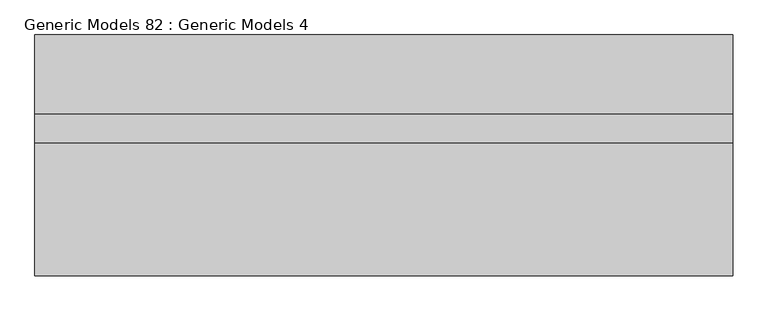
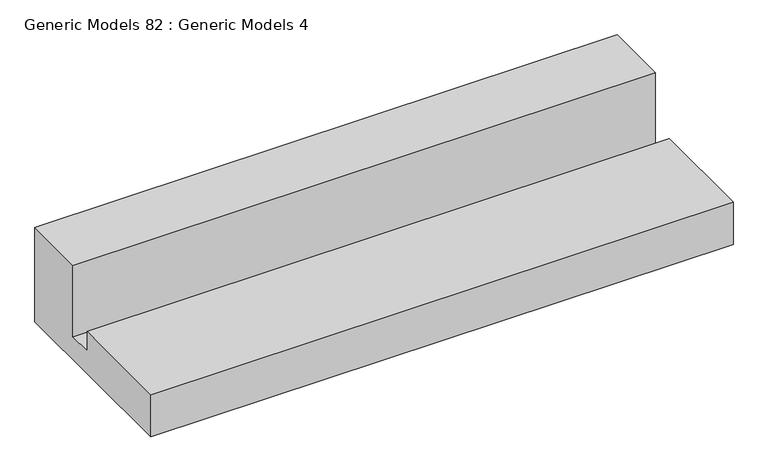
"""IFC4 building model written with IfcOpenShell, lengths in millimetres: proxy geometry, Generic Models 82 : Generic Models 4."""

import ifcopenshell
import ifcopenshell.guid

model = None  # the IFC model being written
_history = None  # IfcOwnerHistory: only IFC2X3 demands one
_inside = {}  # id of a spatial element -> (the spatial element, [elements in it])
_under = {}  # id of a project, library or spatial element -> (it, [spatial elements below it])
_declared = {}  # id of a project -> (the project, [libraries it declares])
_typed = {}  # id of a type object -> (the type object, [elements of that type])
_made_of = {}  # id of a material, layer set ... -> (it, [elements and type objects made of it])


def new_model(schema):
    """Start an empty IFC model of exactly this schema.

    Asked for "IFC4X3", IfcOpenShell would pick the latest addendum, in which some entities
    have other attributes; the version numbers below select the first issue.
    IFC2X3 requires an IfcOwnerHistory on every rooted entity: one is made here for all.
    """
    global model, _history
    if schema == "IFC4X3":
        model = ifcopenshell.file(schema_version=(4, 3, 0, 0))
    else:
        model = ifcopenshell.file(schema=schema)
    _inside.clear()
    _under.clear()
    _declared.clear()
    _typed.clear()
    _made_of.clear()
    _history = None
    if model.schema == "IFC2X3":
        org = make("IfcOrganization", Name="unknown")
        user = make(
            "IfcPersonAndOrganization",
            ThePerson=make("IfcPerson", FamilyName="unknown"),
            TheOrganization=org,
        )
        app = make(
            "IfcApplication",
            ApplicationDeveloper=org,
            Version="unknown",
            ApplicationFullName="unknown",
            ApplicationIdentifier="unknown",
        )
        _history = make(
            "IfcOwnerHistory",
            OwningUser=user,
            OwningApplication=app,
            ChangeAction="ADDED",
            CreationDate=0,
        )
    return model


def make(cls, **values):
    """One entity of the class cls with the attributes given. An attribute that is None is left unset."""
    return model.create_entity(
        cls, **{name: value for name, value in values.items() if value is not None}
    )


def rooted(cls, **values):
    """An entity with a GlobalId (a new one), such as an element, a storey or a relation."""
    return make(cls, GlobalId=ifcopenshell.guid.new(), OwnerHistory=_history, **values)


def si_unit(unit_type, name, prefix=None):
    """IfcSIUnit, for example si_unit("LENGTHUNIT", "METRE", prefix="MILLI")."""
    return make("IfcSIUnit", UnitType=unit_type, Prefix=prefix, Name=name)


def assignment(units):
    """IfcUnitAssignment: the units of a project."""
    return None if units is None else make("IfcUnitAssignment", Units=units)


def point(xyz):
    """IfcCartesianPoint."""
    return None if xyz is None else make("IfcCartesianPoint", Coordinates=xyz)


def direction(xyz):
    """IfcDirection."""
    return None if xyz is None else make("IfcDirection", DirectionRatios=xyz)


def frame(location, z_axis=None, x_axis=None):
    """IfcAxis2Placement3D, a coordinate frame: its origin and axes. An axis left out is left unset."""
    return make(
        "IfcAxis2Placement3D",
        Location=point(location),
        Axis=direction(z_axis),
        RefDirection=direction(x_axis),
    )


def origin():
    """The frame at (0, 0, 0) with its axes left unset."""
    return frame((0.0, 0.0, 0.0))


def place(relative_to, where):
    """IfcLocalPlacement: puts the frame where relative to a parent placement (None: the world)."""
    return make(
        "IfcLocalPlacement", PlacementRelTo=relative_to, RelativePlacement=where
    )


def context(
    kind, dimensions, precision=None, world=None, true_north=None, identifier=None
):
    """IfcGeometricRepresentationContext, for example the 3D "Model" context."""
    return make(
        "IfcGeometricRepresentationContext",
        ContextIdentifier=identifier,
        ContextType=kind,
        CoordinateSpaceDimension=dimensions,
        Precision=precision,
        WorldCoordinateSystem=world,
        TrueNorth=true_north,
    )


def project(units=None, contexts=None):
    """IfcProject with its units and contexts."""
    return rooted(
        "IfcProject",
        Name="project",
        RepresentationContexts=contexts,
        UnitsInContext=assignment(units),
    )


def spatial(cls, under=None, at=None, **own):
    """A site, building, storey or space (cls), placed at a placement, below another one or the project."""
    s = rooted(cls, ObjectPlacement=at, **own)
    if under is not None:
        _under.setdefault(under.id(), (under, []))[1].append(s)
    return s


def polyline(points):
    """IfcPolyline through the points."""
    return make("IfcPolyline", Points=[point(p) for p in points])


def outline(outer, holes=None, kind="AREA"):
    """IfcArbitraryClosedProfileDef: a profile drawn as a closed curve; with holes, ...WithVoids."""
    if holes is None:
        return make("IfcArbitraryClosedProfileDef", ProfileType=kind, OuterCurve=outer)
    return make(
        "IfcArbitraryProfileDefWithVoids",
        ProfileType=kind,
        OuterCurve=outer,
        InnerCurves=holes,
    )


def extrude(swept, where, along, depth):
    """IfcExtrudedAreaSolid: the profile swept, set in the frame where, extruded along a direction by depth."""
    return make(
        "IfcExtrudedAreaSolid",
        SweptArea=swept,
        Position=where,
        ExtrudedDirection=direction(along),
        Depth=depth,
    )


def shape(context_of_items, identifier, shape_type, items):
    """IfcShapeRepresentation: the items that make up one representation, for example the "Body"."""
    return make(
        "IfcShapeRepresentation",
        ContextOfItems=context_of_items,
        RepresentationIdentifier=identifier,
        RepresentationType=shape_type,
        Items=items,
    )


def source(mapping_origin, context_of_items, identifier, shape_type, items):
    """IfcRepresentationMap: a shape defined once, which mapped items show again and again."""
    return make(
        "IfcRepresentationMap",
        MappingOrigin=mapping_origin,
        MappedRepresentation=shape(context_of_items, identifier, shape_type, items),
    )


def transform(
    local_origin,
    x_axis=None,
    y_axis=None,
    z_axis=None,
    scale=None,
    scale2=None,
    scale3=None,
    uniform=True,
):
    """IfcCartesianTransformationOperator3D, or its non-uniform kind. x_axis, y_axis, z_axis: its Axis1, 2, 3."""
    if uniform:
        return make(
            "IfcCartesianTransformationOperator3D",
            Axis1=direction(x_axis),
            Axis2=direction(y_axis),
            LocalOrigin=point(local_origin),
            Scale=scale,
            Axis3=direction(z_axis),
        )
    return make(
        "IfcCartesianTransformationOperator3DnonUniform",
        Axis1=direction(x_axis),
        Axis2=direction(y_axis),
        LocalOrigin=point(local_origin),
        Scale=scale,
        Axis3=direction(z_axis),
        Scale2=scale2,
        Scale3=scale3,
    )


def mapped(mapping_source, mapping_target):
    """IfcMappedItem: shows the shape of a source again, moved by a transform."""
    return make(
        "IfcMappedItem", MappingSource=mapping_source, MappingTarget=mapping_target
    )


def made_of(thing, what):
    """Note that an element or type object is made of a material, layer set ...; save() writes the relation."""
    if what is not None:
        _made_of.setdefault(what.id(), (what, []))[1].append(thing)
    return thing


def element(
    cls,
    number,
    at=None,
    inside=None,
    cuts=None,
    type_object=None,
    material=None,
    context=None,
    identifier="Body",
    shape_type=None,
    held_by="IfcProductDefinitionShape",
    body=None,
    shapes=None,
    **own,
):
    """One element of the class cls, such as IfcWall. Its Tag is "e" and its number.

    at: its placement. inside: the storey or other place that contains it. cuts: it is an
    opening in that element (IfcRelVoidsElement). A single representation is given by context,
    identifier, shape_type and body (its items); several are given by shapes. held_by: the class
    of the entity that holds the representations. save() writes the other relations.
    """
    e = rooted(cls, Tag="e%d" % number, ObjectPlacement=at, **own)
    if body is not None:
        shapes = [shape(context, identifier, shape_type, body)]
    if shapes is not None:
        e.Representation = make(held_by, Representations=shapes)
    if inside is not None:
        _inside.setdefault(inside.id(), (inside, []))[1].append(e)
    if cuts is not None:
        rooted(
            "IfcRelVoidsElement", RelatingBuildingElement=cuts, RelatedOpeningElement=e
        )
    if type_object is not None:
        _typed.setdefault(type_object.id(), (type_object, []))[1].append(e)
    return made_of(e, material)


def aggregate(whole, parts):
    """IfcRelAggregates: a whole, such as a stair, and the parts it consists of."""
    return rooted("IfcRelAggregates", RelatingObject=whole, RelatedObjects=parts)


def save(model, path):
    """Write the relations noted so far, then the file.

    IfcRelAggregates (storeys below a building ...), IfcRelContainedInSpatialStructure (elements
    in a storey), IfcRelDefinesByType, IfcRelAssociatesMaterial and IfcRelDeclares: one each for
    every whole, place, type object, material and project.
    """
    for whole, parts in _under.values():
        aggregate(whole, parts)
    for where, things in _inside.values():
        rooted(
            "IfcRelContainedInSpatialStructure",
            RelatedElements=things,
            RelatingStructure=where,
        )
    for kind, things in _typed.values():
        rooted("IfcRelDefinesByType", RelatedObjects=things, RelatingType=kind)
    for what, things in _made_of.values():
        rooted("IfcRelAssociatesMaterial", RelatedObjects=things, RelatingMaterial=what)
    for by, libraries in _declared.values():
        rooted("IfcRelDeclares", RelatingContext=by, RelatedDefinitions=libraries)
    model.write(path)


def generic_models_82_generic_models_4_5136586e(model_context):
    return source(origin(), model_context, "Body", "SweptSolid", [
        extrude(outline(polyline([(-6325.6058624, 123448.5085), (-6325.6058624, 122621.9016693), (-7988.8730338, 122621.9016693), (-7988.8730338, 122992.896), (-7074.4730338, 122992.896), (-7074.4730338, 122820.073267), (-6871.2730338, 122820.073267), (-6871.2730338, 123448.5085), (-6325.6058624, 123448.5085)])), frame((2196.9263704, 0.0, 0.0), z_axis=(1.0, 0.0, 0.0), x_axis=(0.0, 1.0, 0.0)), (0.0, 0.0, 1.0), 4818.3290223),
    ])


if __name__ == "__main__":
    model = new_model("IFC4")
    model_context = context("Model", 3, world=origin())
    ifc_project = project(units=[si_unit("LENGTHUNIT", "METRE", prefix="MILLI")], contexts=[model_context])
    site = spatial("IfcSite", under=ifc_project)
    building = spatial("IfcBuilding", under=site)
    placement = place(None, origin())
    generic_models_82_generic_models_4_shape = generic_models_82_generic_models_4_5136586e(model_context)
    element("IfcBuildingElementProxy", 1, Name="Generic Models 82 : Generic Models 4", ObjectType="Generic Models 82 : Generic Models 4", at=placement, inside=building, context=model_context, shape_type="MappedRepresentation", body=[
        mapped(generic_models_82_generic_models_4_shape, transform((0.0, 0.0, 0.0), x_axis=(1.0, 0.0, 0.0), y_axis=(0.0, 1.0, 0.0), z_axis=(0.0, 0.0, 1.0))),
    ])
    save(model, "model.ifc")

# Revit data of these elements
# Element 1 (IfcBuildingElementProxy, "Generic Models 82 : Generic Models 4")
#   Materials on its faces: "_COMPACTED GRADE"
# Materials
#   "_COMPACTED GRADE": class "Generic", colour RGB 120 100 58, transparency 0, Cost = 0
